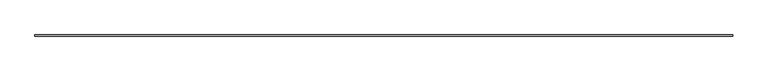
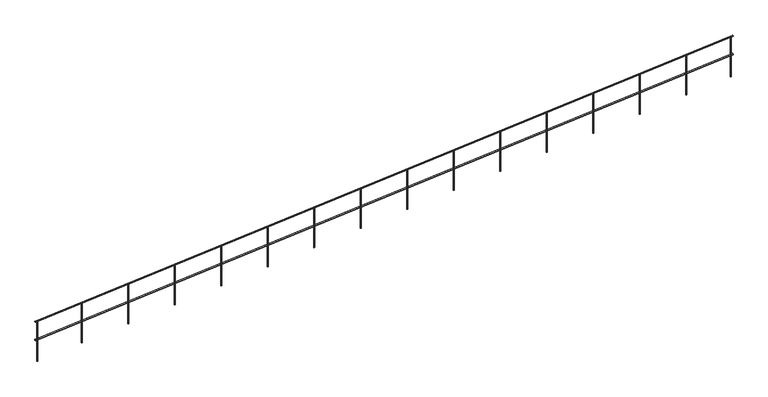
"""IFC4 building model written with IfcOpenShell, lengths in millimetres: railing geometry."""

from ifc_helpers import new_model, si_unit, frame, origin, place, context, project, spatial, ellipse_curve, source, transform, mapped, element, save
from ifc_brep_helpers import plane_surface, cylinder_surface, advanced_brep


def railing_0761552e(model_context):
    return source(origin(), model_context, "Body", "AdvancedBrep", [
        advanced_brep(
        [(42716.32048, 71467.0208589, -615.0519932), (42716.32048, 71437.0208589, -615.0519932), (60716.32048, 71467.0208589, 884.9480068), (60716.32048, 71437.0208589, 884.9480068)],
        [
            (0, 1, ellipse_curve(frame((42716.32048, 71452.0208589, -615.0519932), z_axis=(-1.0, 0.0, 0.0), x_axis=(0.0, 0.0, -0.9999999999999999)), 15.0519932, 15.0)),
            (1, 0, ellipse_curve(frame((42716.32048, 71452.0208589, -615.0519932), z_axis=(-1.0, 0.0, 0.0), x_axis=(0.0, 0.0, -0.9999999999999999)), 15.0519932, 15.0)),
            (2, 3, ellipse_curve(frame((60716.32048, 71452.0208589, 884.9480068), z_axis=(1.0, 0.0, 0.0), x_axis=(0.0, 0.0, -0.9999999999999999)), 15.0519932, 15.0)),
            (3, 2, ellipse_curve(frame((60716.32048, 71452.0208589, 884.9480068), z_axis=(1.0, 0.0, 0.0), x_axis=(0.0, 0.0, -0.9999999999999999)), 15.0519932, 15.0)),
            (0, 2),
            (3, 1),
        ],
        [
            plane_surface(frame((42716.32048, 71452.0208589, -600.0), z_axis=(-1.0, 0.0, 0.0), x_axis=(0.0, 1.0, 0.0))),
            plane_surface(frame((60716.32048, 71452.0208589, 900.0), z_axis=(1.0, 0.0, 0.0), x_axis=(0.0, 1.0, 0.0))),
            cylinder_surface(frame((42717.5661622, 71452.0208589, -614.9481864), z_axis=(-0.9965457582448797, 0.0, -0.08304547985373997), x_axis=(0.0, -1.0, 0.0)), 15.0),
        ],
        [
            (0, [[1, 2]]),
            (1, [[3, 4]]),
            (2, [[-1, 5, -4, 6]]),
            (2, [[-2, -6, -3, -5]]),
        ],
    ),
        advanced_brep(
        [(42716.32048, 71467.0208589, -115.0519932), (42716.32048, 71437.0208589, -115.0519932), (60716.32048, 71467.0208589, 1384.9480068), (60716.32048, 71437.0208589, 1384.9480068)],
        [
            (0, 1, ellipse_curve(frame((42716.32048, 71452.0208589, -115.0519932), z_axis=(-1.0, 0.0, 0.0), x_axis=(0.0, 0.0, -0.9999999999999999)), 15.0519932, 15.0)),
            (1, 0, ellipse_curve(frame((42716.32048, 71452.0208589, -115.0519932), z_axis=(-1.0, 0.0, 0.0), x_axis=(0.0, 0.0, -0.9999999999999999)), 15.0519932, 15.0)),
            (2, 3, ellipse_curve(frame((60716.32048, 71452.0208589, 1384.9480068), z_axis=(1.0, 0.0, 0.0), x_axis=(0.0, 0.0, -0.9999999999999999)), 15.0519932, 15.0)),
            (3, 2, ellipse_curve(frame((60716.32048, 71452.0208589, 1384.9480068), z_axis=(1.0, 0.0, 0.0), x_axis=(0.0, 0.0, -0.9999999999999999)), 15.0519932, 15.0)),
            (0, 2),
            (3, 1),
        ],
        [
            plane_surface(frame((42716.32048, 71452.0208589, -100.0), z_axis=(-1.0, 0.0, 0.0), x_axis=(0.0, 1.0, 0.0))),
            plane_surface(frame((60716.32048, 71452.0208589, 1400.0), z_axis=(1.0, 0.0, 0.0), x_axis=(0.0, 1.0, 0.0))),
            cylinder_surface(frame((42717.5661622, 71452.0208589, -114.9481864), z_axis=(-0.9965457582448797, 0.0, -0.08304547985373997), x_axis=(0.0, -1.0, 0.0)), 15.0),
        ],
        [
            (0, [[1, 2]]),
            (1, [[3, 4]]),
            (2, [[-1, 5, -4, 6]]),
            (2, [[-2, -6, -3, -5]]),
        ],
    ),
        advanced_brep(
        [(59516.32048, 71437.0208589, 1269.8960136), (59516.32048, 71437.0208589, 200.0), (59516.32048, 71467.0208589, 200.0), (59516.32048, 71467.0208589, 1269.8960136)],
        [
            (0, 1),
            (1, 2, ellipse_curve(frame((59516.32048, 71452.0208589, 200.0), z_axis=(-0.08304547985373996, 0.0, 0.9965457582448797), x_axis=(0.9965457582448798, 0.0, 0.08304547985373881)), 15.0519932, 15.0)),
            (2, 3),
            (3, 0, ellipse_curve(frame((59516.32048, 71452.0208589, 1269.8960136), z_axis=(0.083045479853741, 0.0, -0.9965457582448796), x_axis=(0.9965457582448797, 0.0, 0.08304547985374044)), 15.0519932, 15.0)),
            (0, 3, ellipse_curve(frame((59516.32048, 71452.0208589, 1269.8960136), z_axis=(0.083045479853741, 0.0, -0.9965457582448796), x_axis=(0.9965457582448797, 0.0, 0.08304547985374044)), 15.0519932, 15.0)),
            (2, 1, ellipse_curve(frame((59516.32048, 71452.0208589, 200.0), z_axis=(-0.08304547985373996, 0.0, 0.9965457582448797), x_axis=(0.9965457582448798, 0.0, 0.08304547985373881)), 15.0519932, 15.0)),
        ],
        [
            cylinder_surface(frame((59516.32048, 71452.0208589, 100.0), z_axis=(0.0, 0.0, 1.0), x_axis=(0.0, 1.0, 0.0)), 15.0),
            plane_surface(frame((59541.32048, 71477.0208589, 1271.9793469), z_axis=(-0.083045479853741, 0.0, 0.9965457582448796), x_axis=(0.0, -1.0, 0.0))),
            plane_surface(frame((59491.32048, 71477.0208589, 197.9166667), z_axis=(0.08304547985373996, 0.0, -0.9965457582448797), x_axis=(0.0, -1.0, 0.0))),
        ],
        [
            (0, [[1, 2, 3, 4]]),
            (0, [[-1, 5, -3, 6]]),
            (1, [[-4, -5]]),
            (2, [[-2, -6]]),
        ],
    ),
        advanced_brep(
        [(58316.32048, 71437.0208589, 1169.8960136), (58316.32048, 71437.0208589, 100.0), (58316.32048, 71467.0208589, 100.0), (58316.32048, 71467.0208589, 1169.8960136)],
        [
            (0, 1),
            (1, 2, ellipse_curve(frame((58316.32048, 71452.0208589, 100.0), z_axis=(-0.08304547985373996, 0.0, 0.9965457582448797), x_axis=(0.9965457582448798, 0.0, 0.08304547985373881)), 15.0519932, 15.0)),
            (2, 3),
            (3, 0, ellipse_curve(frame((58316.32048, 71452.0208589, 1169.8960136), z_axis=(0.083045479853741, 0.0, -0.9965457582448796), x_axis=(0.9965457582448797, 0.0, 0.08304547985374044)), 15.0519932, 15.0)),
            (0, 3, ellipse_curve(frame((58316.32048, 71452.0208589, 1169.8960136), z_axis=(0.083045479853741, 0.0, -0.9965457582448796), x_axis=(0.9965457582448797, 0.0, 0.08304547985374044)), 15.0519932, 15.0)),
            (2, 1, ellipse_curve(frame((58316.32048, 71452.0208589, 100.0), z_axis=(-0.08304547985373996, 0.0, 0.9965457582448797), x_axis=(0.9965457582448798, 0.0, 0.08304547985373881)), 15.0519932, 15.0)),
        ],
        [
            cylinder_surface(frame((58316.32048, 71452.0208589, 0.0), z_axis=(0.0, 0.0, 1.0), x_axis=(0.0, 1.0, 0.0)), 15.0),
            plane_surface(frame((58341.32048, 71477.0208589, 1171.9793469), z_axis=(-0.083045479853741, 0.0, 0.9965457582448796), x_axis=(0.0, -1.0, 0.0))),
            plane_surface(frame((58291.32048, 71477.0208589, 97.9166667), z_axis=(0.08304547985373996, 0.0, -0.9965457582448797), x_axis=(0.0, -1.0, 0.0))),
        ],
        [
            (0, [[1, 2, 3, 4]]),
            (0, [[-1, 5, -3, 6]]),
            (1, [[-4, -5]]),
            (2, [[-2, -6]]),
        ],
    ),
        advanced_brep(
        [(57116.32048, 71437.0208589, 1069.8960136), (57116.32048, 71437.0208589, 0.0), (57116.32048, 71467.0208589, 0.0), (57116.32048, 71467.0208589, 1069.8960136)],
        [
            (0, 1),
            (1, 2, ellipse_curve(frame((57116.32048, 71452.0208589, 0.0), z_axis=(-0.08304547985373996, 0.0, 0.9965457582448797), x_axis=(0.9965457582448798, 0.0, 0.08304547985373881)), 15.0519932, 15.0)),
            (2, 3),
            (3, 0, ellipse_curve(frame((57116.32048, 71452.0208589, 1069.8960136), z_axis=(0.083045479853741, 0.0, -0.9965457582448796), x_axis=(0.9965457582448797, 0.0, 0.08304547985374044)), 15.0519932, 15.0)),
            (0, 3, ellipse_curve(frame((57116.32048, 71452.0208589, 1069.8960136), z_axis=(0.083045479853741, 0.0, -0.9965457582448796), x_axis=(0.9965457582448797, 0.0, 0.08304547985374044)), 15.0519932, 15.0)),
            (2, 1, ellipse_curve(frame((57116.32048, 71452.0208589, 0.0), z_axis=(-0.08304547985373996, 0.0, 0.9965457582448797), x_axis=(0.9965457582448798, 0.0, 0.08304547985373881)), 15.0519932, 15.0)),
        ],
        [
            cylinder_surface(frame((57116.32048, 71452.0208589, -100.0), z_axis=(0.0, 0.0, 1.0), x_axis=(0.0, 1.0, 0.0)), 15.0),
            plane_surface(frame((57141.32048, 71477.0208589, 1071.9793469), z_axis=(-0.083045479853741, 0.0, 0.9965457582448796), x_axis=(0.0, -1.0, 0.0))),
            plane_surface(frame((57091.32048, 71477.0208589, -2.0833333), z_axis=(0.08304547985373996, 0.0, -0.9965457582448797), x_axis=(0.0, -1.0, 0.0))),
        ],
        [
            (0, [[1, 2, 3, 4]]),
            (0, [[-1, 5, -3, 6]]),
            (1, [[-4, -5]]),
            (2, [[-2, -6]]),
        ],
    ),
        advanced_brep(
        [(55916.32048, 71437.0208589, 969.8960136), (55916.32048, 71437.0208589, -100.0), (55916.32048, 71467.0208589, -100.0), (55916.32048, 71467.0208589, 969.8960136)],
        [
            (0, 1),
            (1, 2, ellipse_curve(frame((55916.32048, 71452.0208589, -100.0), z_axis=(-0.08304547985373996, 0.0, 0.9965457582448797), x_axis=(0.9965457582448798, 0.0, 0.08304547985373881)), 15.0519932, 15.0)),
            (2, 3),
            (3, 0, ellipse_curve(frame((55916.32048, 71452.0208589, 969.8960136), z_axis=(0.083045479853741, 0.0, -0.9965457582448796), x_axis=(0.9965457582448797, 0.0, 0.08304547985374044)), 15.0519932, 15.0)),
            (0, 3, ellipse_curve(frame((55916.32048, 71452.0208589, 969.8960136), z_axis=(0.083045479853741, 0.0, -0.9965457582448796), x_axis=(0.9965457582448797, 0.0, 0.08304547985374044)), 15.0519932, 15.0)),
            (2, 1, ellipse_curve(frame((55916.32048, 71452.0208589, -100.0), z_axis=(-0.08304547985373996, 0.0, 0.9965457582448797), x_axis=(0.9965457582448798, 0.0, 0.08304547985373881)), 15.0519932, 15.0)),
        ],
        [
            cylinder_surface(frame((55916.32048, 71452.0208589, -200.0), z_axis=(0.0, 0.0, 1.0), x_axis=(0.0, 1.0, 0.0)), 15.0),
            plane_surface(frame((55941.32048, 71477.0208589, 971.9793469), z_axis=(-0.083045479853741, 0.0, 0.9965457582448796), x_axis=(0.0, -1.0, 0.0))),
            plane_surface(frame((55891.32048, 71477.0208589, -102.0833333), z_axis=(0.08304547985373996, 0.0, -0.9965457582448797), x_axis=(0.0, -1.0, 0.0))),
        ],
        [
            (0, [[1, 2, 3, 4]]),
            (0, [[-1, 5, -3, 6]]),
            (1, [[-4, -5]]),
            (2, [[-2, -6]]),
        ],
    ),
        advanced_brep(
        [(54716.32048, 71437.0208589, 869.8960136), (54716.32048, 71437.0208589, -200.0), (54716.32048, 71467.0208589, -200.0), (54716.32048, 71467.0208589, 869.8960136)],
        [
            (0, 1),
            (1, 2, ellipse_curve(frame((54716.32048, 71452.0208589, -200.0), z_axis=(-0.08304547985373996, 0.0, 0.9965457582448797), x_axis=(0.9965457582448798, 0.0, 0.08304547985373881)), 15.0519932, 15.0)),
            (2, 3),
            (3, 0, ellipse_curve(frame((54716.32048, 71452.0208589, 869.8960136), z_axis=(0.083045479853741, 0.0, -0.9965457582448796), x_axis=(0.9965457582448797, 0.0, 0.08304547985374044)), 15.0519932, 15.0)),
            (0, 3, ellipse_curve(frame((54716.32048, 71452.0208589, 869.8960136), z_axis=(0.083045479853741, 0.0, -0.9965457582448796), x_axis=(0.9965457582448797, 0.0, 0.08304547985374044)), 15.0519932, 15.0)),
            (2, 1, ellipse_curve(frame((54716.32048, 71452.0208589, -200.0), z_axis=(-0.08304547985373996, 0.0, 0.9965457582448797), x_axis=(0.9965457582448798, 0.0, 0.08304547985373881)), 15.0519932, 15.0)),
        ],
        [
            cylinder_surface(frame((54716.32048, 71452.0208589, -300.0), z_axis=(0.0, 0.0, 1.0), x_axis=(0.0, 1.0, 0.0)), 15.0),
            plane_surface(frame((54741.32048, 71477.0208589, 871.9793469), z_axis=(-0.083045479853741, 0.0, 0.9965457582448796), x_axis=(0.0, -1.0, 0.0))),
            plane_surface(frame((54691.32048, 71477.0208589, -202.0833333), z_axis=(0.08304547985373996, 0.0, -0.9965457582448797), x_axis=(0.0, -1.0, 0.0))),
        ],
        [
            (0, [[1, 2, 3, 4]]),
            (0, [[-1, 5, -3, 6]]),
            (1, [[-4, -5]]),
            (2, [[-2, -6]]),
        ],
    ),
        advanced_brep(
        [(53516.32048, 71437.0208589, 769.8960136), (53516.32048, 71437.0208589, -300.0), (53516.32048, 71467.0208589, -300.0), (53516.32048, 71467.0208589, 769.8960136)],
        [
            (0, 1),
            (1, 2, ellipse_curve(frame((53516.32048, 71452.0208589, -300.0), z_axis=(-0.08304547985373996, 0.0, 0.9965457582448797), x_axis=(0.9965457582448798, 0.0, 0.08304547985373881)), 15.0519932, 15.0)),
            (2, 3),
            (3, 0, ellipse_curve(frame((53516.32048, 71452.0208589, 769.8960136), z_axis=(0.083045479853741, 0.0, -0.9965457582448796), x_axis=(0.9965457582448797, 0.0, 0.08304547985374044)), 15.0519932, 15.0)),
            (0, 3, ellipse_curve(frame((53516.32048, 71452.0208589, 769.8960136), z_axis=(0.083045479853741, 0.0, -0.9965457582448796), x_axis=(0.9965457582448797, 0.0, 0.08304547985374044)), 15.0519932, 15.0)),
            (2, 1, ellipse_curve(frame((53516.32048, 71452.0208589, -300.0), z_axis=(-0.08304547985373996, 0.0, 0.9965457582448797), x_axis=(0.9965457582448798, 0.0, 0.08304547985373881)), 15.0519932, 15.0)),
        ],
        [
            cylinder_surface(frame((53516.32048, 71452.0208589, -400.0), z_axis=(0.0, 0.0, 1.0), x_axis=(0.0, 1.0, 0.0)), 15.0),
            plane_surface(frame((53541.32048, 71477.0208589, 771.9793469), z_axis=(-0.083045479853741, 0.0, 0.9965457582448796), x_axis=(0.0, -1.0, 0.0))),
            plane_surface(frame((53491.32048, 71477.0208589, -302.0833333), z_axis=(0.08304547985373996, 0.0, -0.9965457582448797), x_axis=(0.0, -1.0, 0.0))),
        ],
        [
            (0, [[1, 2, 3, 4]]),
            (0, [[-1, 5, -3, 6]]),
            (1, [[-4, -5]]),
            (2, [[-2, -6]]),
        ],
    ),
        advanced_brep(
        [(52316.32048, 71437.0208589, 669.8960136), (52316.32048, 71437.0208589, -400.0), (52316.32048, 71467.0208589, -400.0), (52316.32048, 71467.0208589, 669.8960136)],
        [
            (0, 1),
            (1, 2, ellipse_curve(frame((52316.32048, 71452.0208589, -400.0), z_axis=(-0.08304547985373996, 0.0, 0.9965457582448797), x_axis=(0.9965457582448798, 0.0, 0.08304547985373881)), 15.0519932, 15.0)),
            (2, 3),
            (3, 0, ellipse_curve(frame((52316.32048, 71452.0208589, 669.8960136), z_axis=(0.083045479853741, 0.0, -0.9965457582448796), x_axis=(0.9965457582448797, 0.0, 0.08304547985374044)), 15.0519932, 15.0)),
            (0, 3, ellipse_curve(frame((52316.32048, 71452.0208589, 669.8960136), z_axis=(0.083045479853741, 0.0, -0.9965457582448796), x_axis=(0.9965457582448797, 0.0, 0.08304547985374044)), 15.0519932, 15.0)),
            (2, 1, ellipse_curve(frame((52316.32048, 71452.0208589, -400.0), z_axis=(-0.08304547985373996, 0.0, 0.9965457582448797), x_axis=(0.9965457582448798, 0.0, 0.08304547985373881)), 15.0519932, 15.0)),
        ],
        [
            cylinder_surface(frame((52316.32048, 71452.0208589, -500.0), z_axis=(0.0, 0.0, 1.0), x_axis=(0.0, 1.0, 0.0)), 15.0),
            plane_surface(frame((52341.32048, 71477.0208589, 671.9793469), z_axis=(-0.083045479853741, 0.0, 0.9965457582448796), x_axis=(0.0, -1.0, 0.0))),
            plane_surface(frame((52291.32048, 71477.0208589, -402.0833333), z_axis=(0.08304547985373996, 0.0, -0.9965457582448797), x_axis=(0.0, -1.0, 0.0))),
        ],
        [
            (0, [[1, 2, 3, 4]]),
            (0, [[-1, 5, -3, 6]]),
            (1, [[-4, -5]]),
            (2, [[-2, -6]]),
        ],
    ),
        advanced_brep(
        [(51116.32048, 71437.0208589, 569.8960136), (51116.32048, 71437.0208589, -500.0), (51116.32048, 71467.0208589, -500.0), (51116.32048, 71467.0208589, 569.8960136)],
        [
            (0, 1),
            (1, 2, ellipse_curve(frame((51116.32048, 71452.0208589, -500.0), z_axis=(-0.08304547985373996, 0.0, 0.9965457582448797), x_axis=(0.9965457582448798, 0.0, 0.08304547985373881)), 15.0519932, 15.0)),
            (2, 3),
            (3, 0, ellipse_curve(frame((51116.32048, 71452.0208589, 569.8960136), z_axis=(0.083045479853741, 0.0, -0.9965457582448796), x_axis=(0.9965457582448797, 0.0, 0.08304547985374044)), 15.0519932, 15.0)),
            (0, 3, ellipse_curve(frame((51116.32048, 71452.0208589, 569.8960136), z_axis=(0.083045479853741, 0.0, -0.9965457582448796), x_axis=(0.9965457582448797, 0.0, 0.08304547985374044)), 15.0519932, 15.0)),
            (2, 1, ellipse_curve(frame((51116.32048, 71452.0208589, -500.0), z_axis=(-0.08304547985373996, 0.0, 0.9965457582448797), x_axis=(0.9965457582448798, 0.0, 0.08304547985373881)), 15.0519932, 15.0)),
        ],
        [
            cylinder_surface(frame((51116.32048, 71452.0208589, -600.0), z_axis=(0.0, 0.0, 1.0), x_axis=(0.0, 1.0, 0.0)), 15.0),
            plane_surface(frame((51141.32048, 71477.0208589, 571.9793469), z_axis=(-0.083045479853741, 0.0, 0.9965457582448796), x_axis=(0.0, -1.0, 0.0))),
            plane_surface(frame((51091.32048, 71477.0208589, -502.0833333), z_axis=(0.08304547985373996, 0.0, -0.9965457582448797), x_axis=(0.0, -1.0, 0.0))),
        ],
        [
            (0, [[1, 2, 3, 4]]),
            (0, [[-1, 5, -3, 6]]),
            (1, [[-4, -5]]),
            (2, [[-2, -6]]),
        ],
    ),
        advanced_brep(
        [(49916.32048, 71437.0208589, 469.8960136), (49916.32048, 71437.0208589, -600.0), (49916.32048, 71467.0208589, -600.0), (49916.32048, 71467.0208589, 469.8960136)],
        [
            (0, 1),
            (1, 2, ellipse_curve(frame((49916.32048, 71452.0208589, -600.0), z_axis=(-0.08304547985373996, 0.0, 0.9965457582448797), x_axis=(0.9965457582448798, 0.0, 0.08304547985373881)), 15.0519932, 15.0)),
            (2, 3),
            (3, 0, ellipse_curve(frame((49916.32048, 71452.0208589, 469.8960136), z_axis=(0.083045479853741, 0.0, -0.9965457582448796), x_axis=(0.9965457582448797, 0.0, 0.08304547985374044)), 15.0519932, 15.0)),
            (0, 3, ellipse_curve(frame((49916.32048, 71452.0208589, 469.8960136), z_axis=(0.083045479853741, 0.0, -0.9965457582448796), x_axis=(0.9965457582448797, 0.0, 0.08304547985374044)), 15.0519932, 15.0)),
            (2, 1, ellipse_curve(frame((49916.32048, 71452.0208589, -600.0), z_axis=(-0.08304547985373996, 0.0, 0.9965457582448797), x_axis=(0.9965457582448798, 0.0, 0.08304547985373881)), 15.0519932, 15.0)),
        ],
        [
            cylinder_surface(frame((49916.32048, 71452.0208589, -700.0), z_axis=(0.0, 0.0, 1.0), x_axis=(0.0, 1.0, 0.0)), 15.0),
            plane_surface(frame((49941.32048, 71477.0208589, 471.9793469), z_axis=(-0.083045479853741, 0.0, 0.9965457582448796), x_axis=(0.0, -1.0, 0.0))),
            plane_surface(frame((49891.32048, 71477.0208589, -602.0833333), z_axis=(0.08304547985373996, 0.0, -0.9965457582448797), x_axis=(0.0, -1.0, 0.0))),
        ],
        [
            (0, [[1, 2, 3, 4]]),
            (0, [[-1, 5, -3, 6]]),
            (1, [[-4, -5]]),
            (2, [[-2, -6]]),
        ],
    ),
        advanced_brep(
        [(48716.32048, 71437.0208589, 369.8960136), (48716.32048, 71437.0208589, -700.0), (48716.32048, 71467.0208589, -700.0), (48716.32048, 71467.0208589, 369.8960136)],
        [
            (0, 1),
            (1, 2, ellipse_curve(frame((48716.32048, 71452.0208589, -700.0), z_axis=(-0.08304547985373996, 0.0, 0.9965457582448797), x_axis=(0.9965457582448798, 0.0, 0.08304547985373881)), 15.0519932, 15.0)),
            (2, 3),
            (3, 0, ellipse_curve(frame((48716.32048, 71452.0208589, 369.8960136), z_axis=(0.083045479853741, 0.0, -0.9965457582448796), x_axis=(0.9965457582448797, 0.0, 0.08304547985374044)), 15.0519932, 15.0)),
            (0, 3, ellipse_curve(frame((48716.32048, 71452.0208589, 369.8960136), z_axis=(0.083045479853741, 0.0, -0.9965457582448796), x_axis=(0.9965457582448797, 0.0, 0.08304547985374044)), 15.0519932, 15.0)),
            (2, 1, ellipse_curve(frame((48716.32048, 71452.0208589, -700.0), z_axis=(-0.08304547985373996, 0.0, 0.9965457582448797), x_axis=(0.9965457582448798, 0.0, 0.08304547985373881)), 15.0519932, 15.0)),
        ],
        [
            cylinder_surface(frame((48716.32048, 71452.0208589, -800.0), z_axis=(0.0, 0.0, 1.0), x_axis=(0.0, 1.0, 0.0)), 15.0),
            plane_surface(frame((48741.32048, 71477.0208589, 371.9793469), z_axis=(-0.083045479853741, 0.0, 0.9965457582448796), x_axis=(0.0, -1.0, 0.0))),
            plane_surface(frame((48691.32048, 71477.0208589, -702.0833333), z_axis=(0.08304547985373996, 0.0, -0.9965457582448797), x_axis=(0.0, -1.0, 0.0))),
        ],
        [
            (0, [[1, 2, 3, 4]]),
            (0, [[-1, 5, -3, 6]]),
            (1, [[-4, -5]]),
            (2, [[-2, -6]]),
        ],
    ),
        advanced_brep(
        [(47516.32048, 71437.0208589, 269.8960136), (47516.32048, 71437.0208589, -800.0), (47516.32048, 71467.0208589, -800.0), (47516.32048, 71467.0208589, 269.8960136)],
        [
            (0, 1),
            (1, 2, ellipse_curve(frame((47516.32048, 71452.0208589, -800.0), z_axis=(-0.08304547985373996, 0.0, 0.9965457582448797), x_axis=(0.9965457582448798, 0.0, 0.08304547985373881)), 15.0519932, 15.0)),
            (2, 3),
            (3, 0, ellipse_curve(frame((47516.32048, 71452.0208589, 269.8960136), z_axis=(0.083045479853741, 0.0, -0.9965457582448796), x_axis=(0.9965457582448797, 0.0, 0.08304547985374044)), 15.0519932, 15.0)),
            (0, 3, ellipse_curve(frame((47516.32048, 71452.0208589, 269.8960136), z_axis=(0.083045479853741, 0.0, -0.9965457582448796), x_axis=(0.9965457582448797, 0.0, 0.08304547985374044)), 15.0519932, 15.0)),
            (2, 1, ellipse_curve(frame((47516.32048, 71452.0208589, -800.0), z_axis=(-0.08304547985373996, 0.0, 0.9965457582448797), x_axis=(0.9965457582448798, 0.0, 0.08304547985373881)), 15.0519932, 15.0)),
        ],
        [
            cylinder_surface(frame((47516.32048, 71452.0208589, -900.0), z_axis=(0.0, 0.0, 1.0), x_axis=(0.0, 1.0, 0.0)), 15.0),
            plane_surface(frame((47541.32048, 71477.0208589, 271.9793469), z_axis=(-0.083045479853741, 0.0, 0.9965457582448796), x_axis=(0.0, -1.0, 0.0))),
            plane_surface(frame((47491.32048, 71477.0208589, -802.0833333), z_axis=(0.08304547985373996, 0.0, -0.9965457582448797), x_axis=(0.0, -1.0, 0.0))),
        ],
        [
            (0, [[1, 2, 3, 4]]),
            (0, [[-1, 5, -3, 6]]),
            (1, [[-4, -5]]),
            (2, [[-2, -6]]),
        ],
    ),
        advanced_brep(
        [(46316.32048, 71437.0208589, 169.8960136), (46316.32048, 71437.0208589, -900.0), (46316.32048, 71467.0208589, -900.0), (46316.32048, 71467.0208589, 169.8960136)],
        [
            (0, 1),
            (1, 2, ellipse_curve(frame((46316.32048, 71452.0208589, -900.0), z_axis=(-0.08304547985373996, 0.0, 0.9965457582448797), x_axis=(0.9965457582448798, 0.0, 0.08304547985373881)), 15.0519932, 15.0)),
            (2, 3),
            (3, 0, ellipse_curve(frame((46316.32048, 71452.0208589, 169.8960136), z_axis=(0.083045479853741, 0.0, -0.9965457582448796), x_axis=(0.9965457582448797, 0.0, 0.08304547985374044)), 15.0519932, 15.0)),
            (0, 3, ellipse_curve(frame((46316.32048, 71452.0208589, 169.8960136), z_axis=(0.083045479853741, 0.0, -0.9965457582448796), x_axis=(0.9965457582448797, 0.0, 0.08304547985374044)), 15.0519932, 15.0)),
            (2, 1, ellipse_curve(frame((46316.32048, 71452.0208589, -900.0), z_axis=(-0.08304547985373996, 0.0, 0.9965457582448797), x_axis=(0.9965457582448798, 0.0, 0.08304547985373881)), 15.0519932, 15.0)),
        ],
        [
            cylinder_surface(frame((46316.32048, 71452.0208589, -1000.0), z_axis=(0.0, 0.0, 1.0), x_axis=(0.0, 1.0, 0.0)), 15.0),
            plane_surface(frame((46341.32048, 71477.0208589, 171.9793469), z_axis=(-0.083045479853741, 0.0, 0.9965457582448796), x_axis=(0.0, -1.0, 0.0))),
            plane_surface(frame((46291.32048, 71477.0208589, -902.0833333), z_axis=(0.08304547985373996, 0.0, -0.9965457582448797), x_axis=(0.0, -1.0, 0.0))),
        ],
        [
            (0, [[1, 2, 3, 4]]),
            (0, [[-1, 5, -3, 6]]),
            (1, [[-4, -5]]),
            (2, [[-2, -6]]),
        ],
    ),
        advanced_brep(
        [(45116.32048, 71437.0208589, 69.8960136), (45116.32048, 71437.0208589, -1000.0), (45116.32048, 71467.0208589, -1000.0), (45116.32048, 71467.0208589, 69.8960136)],
        [
            (0, 1),
            (1, 2, ellipse_curve(frame((45116.32048, 71452.0208589, -1000.0), z_axis=(-0.08304547985373996, 0.0, 0.9965457582448797), x_axis=(0.9965457582448798, 0.0, 0.08304547985373881)), 15.0519932, 15.0)),
            (2, 3),
            (3, 0, ellipse_curve(frame((45116.32048, 71452.0208589, 69.8960136), z_axis=(0.083045479853741, 0.0, -0.9965457582448796), x_axis=(0.9965457582448797, 0.0, 0.08304547985374044)), 15.0519932, 15.0)),
            (0, 3, ellipse_curve(frame((45116.32048, 71452.0208589, 69.8960136), z_axis=(0.083045479853741, 0.0, -0.9965457582448796), x_axis=(0.9965457582448797, 0.0, 0.08304547985374044)), 15.0519932, 15.0)),
            (2, 1, ellipse_curve(frame((45116.32048, 71452.0208589, -1000.0), z_axis=(-0.08304547985373996, 0.0, 0.9965457582448797), x_axis=(0.9965457582448798, 0.0, 0.08304547985373881)), 15.0519932, 15.0)),
        ],
        [
            cylinder_surface(frame((45116.32048, 71452.0208589, -1100.0), z_axis=(0.0, 0.0, 1.0), x_axis=(0.0, 1.0, 0.0)), 15.0),
            plane_surface(frame((45141.32048, 71477.0208589, 71.9793469), z_axis=(-0.083045479853741, 0.0, 0.9965457582448796), x_axis=(0.0, -1.0, 0.0))),
            plane_surface(frame((45091.32048, 71477.0208589, -1002.0833333), z_axis=(0.08304547985373996, 0.0, -0.9965457582448797), x_axis=(0.0, -1.0, 0.0))),
        ],
        [
            (0, [[1, 2, 3, 4]]),
            (0, [[-1, 5, -3, 6]]),
            (1, [[-4, -5]]),
            (2, [[-2, -6]]),
        ],
    ),
        advanced_brep(
        [(43916.32048, 71437.0208589, -30.1039864), (43916.32048, 71437.0208589, -1100.0), (43916.32048, 71467.0208589, -1100.0), (43916.32048, 71467.0208589, -30.1039864)],
        [
            (0, 1),
            (1, 2, ellipse_curve(frame((43916.32048, 71452.0208589, -1100.0), z_axis=(-0.08304547985373996, 0.0, 0.9965457582448797), x_axis=(0.9965457582448798, 0.0, 0.08304547985373881)), 15.0519932, 15.0)),
            (2, 3),
            (3, 0, ellipse_curve(frame((43916.32048, 71452.0208589, -30.1039864), z_axis=(0.083045479853741, 0.0, -0.9965457582448796), x_axis=(0.9965457582448797, 0.0, 0.08304547985374044)), 15.0519932, 15.0)),
            (0, 3, ellipse_curve(frame((43916.32048, 71452.0208589, -30.1039864), z_axis=(0.083045479853741, 0.0, -0.9965457582448796), x_axis=(0.9965457582448797, 0.0, 0.08304547985374044)), 15.0519932, 15.0)),
            (2, 1, ellipse_curve(frame((43916.32048, 71452.0208589, -1100.0), z_axis=(-0.08304547985373996, 0.0, 0.9965457582448797), x_axis=(0.9965457582448798, 0.0, 0.08304547985373881)), 15.0519932, 15.0)),
        ],
        [
            cylinder_surface(frame((43916.32048, 71452.0208589, -1200.0), z_axis=(0.0, 0.0, 1.0), x_axis=(0.0, 1.0, 0.0)), 15.0),
            plane_surface(frame((43941.32048, 71477.0208589, -28.0206531), z_axis=(-0.083045479853741, 0.0, 0.9965457582448796), x_axis=(0.0, -1.0, 0.0))),
            plane_surface(frame((43891.32048, 71477.0208589, -1102.0833333), z_axis=(0.08304547985373996, 0.0, -0.9965457582448797), x_axis=(0.0, -1.0, 0.0))),
        ],
        [
            (0, [[1, 2, 3, 4]]),
            (0, [[-1, 5, -3, 6]]),
            (1, [[-4, -5]]),
            (2, [[-2, -6]]),
        ],
    ),
        advanced_brep(
        [(60666.32048, 71437.0208589, 1365.7293469), (60666.32048, 71437.0208589, 295.8333333), (60666.32048, 71467.0208589, 295.8333333), (60666.32048, 71467.0208589, 1365.7293469)],
        [
            (0, 1),
            (1, 2, ellipse_curve(frame((60666.32048, 71452.0208589, 295.8333333), z_axis=(-0.08304547985373996, 0.0, 0.9965457582448797), x_axis=(0.9965457582448798, 0.0, 0.08304547985373881)), 15.0519932, 15.0)),
            (2, 3),
            (3, 0, ellipse_curve(frame((60666.32048, 71452.0208589, 1365.7293469), z_axis=(0.083045479853741, 0.0, -0.9965457582448796), x_axis=(0.9965457582448797, 0.0, 0.08304547985374044)), 15.0519932, 15.0)),
            (0, 3, ellipse_curve(frame((60666.32048, 71452.0208589, 1365.7293469), z_axis=(0.083045479853741, 0.0, -0.9965457582448796), x_axis=(0.9965457582448797, 0.0, 0.08304547985374044)), 15.0519932, 15.0)),
            (2, 1, ellipse_curve(frame((60666.32048, 71452.0208589, 295.8333333), z_axis=(-0.08304547985373996, 0.0, 0.9965457582448797), x_axis=(0.9965457582448798, 0.0, 0.08304547985373881)), 15.0519932, 15.0)),
        ],
        [
            cylinder_surface(frame((60666.32048, 71452.0208589, 195.8333333), z_axis=(0.0, 0.0, 1.0), x_axis=(0.0, 1.0, 0.0)), 15.0),
            plane_surface(frame((60691.32048, 71477.0208589, 1367.8126802), z_axis=(-0.083045479853741, 0.0, 0.9965457582448796), x_axis=(0.0, -1.0, 0.0))),
            plane_surface(frame((60641.32048, 71477.0208589, 293.75), z_axis=(0.08304547985373996, 0.0, -0.9965457582448797), x_axis=(0.0, -1.0, 0.0))),
        ],
        [
            (0, [[1, 2, 3, 4]]),
            (0, [[-1, 5, -3, 6]]),
            (1, [[-4, -5]]),
            (2, [[-2, -6]]),
        ],
    ),
        advanced_brep(
        [(42766.32048, 71437.0208589, -125.9373198), (42766.32048, 71437.0208589, -1195.8333333), (42766.32048, 71467.0208589, -1195.8333333), (42766.32048, 71467.0208589, -125.9373198)],
        [
            (0, 1),
            (1, 2, ellipse_curve(frame((42766.32048, 71452.0208589, -1195.8333333), z_axis=(-0.08304547985373996, 0.0, 0.9965457582448797), x_axis=(0.9965457582448798, 0.0, 0.08304547985373881)), 15.0519932, 15.0)),
            (2, 3),
            (3, 0, ellipse_curve(frame((42766.32048, 71452.0208589, -125.9373198), z_axis=(0.083045479853741, 0.0, -0.9965457582448796), x_axis=(0.9965457582448797, 0.0, 0.08304547985374044)), 15.0519932, 15.0)),
            (0, 3, ellipse_curve(frame((42766.32048, 71452.0208589, -125.9373198), z_axis=(0.083045479853741, 0.0, -0.9965457582448796), x_axis=(0.9965457582448797, 0.0, 0.08304547985374044)), 15.0519932, 15.0)),
            (2, 1, ellipse_curve(frame((42766.32048, 71452.0208589, -1195.8333333), z_axis=(-0.08304547985373996, 0.0, 0.9965457582448797), x_axis=(0.9965457582448798, 0.0, 0.08304547985373881)), 15.0519932, 15.0)),
        ],
        [
            cylinder_surface(frame((42766.32048, 71452.0208589, -1295.8333333), z_axis=(0.0, 0.0, 1.0), x_axis=(0.0, 1.0, 0.0)), 15.0),
            plane_surface(frame((42791.32048, 71477.0208589, -123.8539864), z_axis=(-0.083045479853741, 0.0, 0.9965457582448796), x_axis=(0.0, -1.0, 0.0))),
            plane_surface(frame((42741.32048, 71477.0208589, -1197.9166667), z_axis=(0.08304547985373996, 0.0, -0.9965457582448797), x_axis=(0.0, -1.0, 0.0))),
        ],
        [
            (0, [[1, 2, 3, 4]]),
            (0, [[-1, 5, -3, 6]]),
            (1, [[-4, -5]]),
            (2, [[-2, -6]]),
        ],
    ),
    ])


if __name__ == "__main__":
    model = new_model("IFC4")
    model_context = context("Model", 3, world=origin())
    ifc_project = project(units=[si_unit("LENGTHUNIT", "METRE", prefix="MILLI")], contexts=[model_context])
    site = spatial("IfcSite", under=ifc_project)
    building = spatial("IfcBuilding", under=site)
    placement = place(None, origin())
    railing_shape = railing_0761552e(model_context)
    element("IfcRailing", 1, at=placement, inside=building, context=model_context, shape_type="MappedRepresentation", body=[
        mapped(railing_shape, transform((0.0, 0.0, 0.0), x_axis=(1.0, 0.0, 0.0), y_axis=(0.0, 1.0, 0.0), z_axis=(0.0, 0.0, 1.0))),
    ])
    save(model, "model.ifc")
